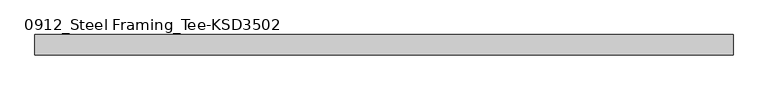
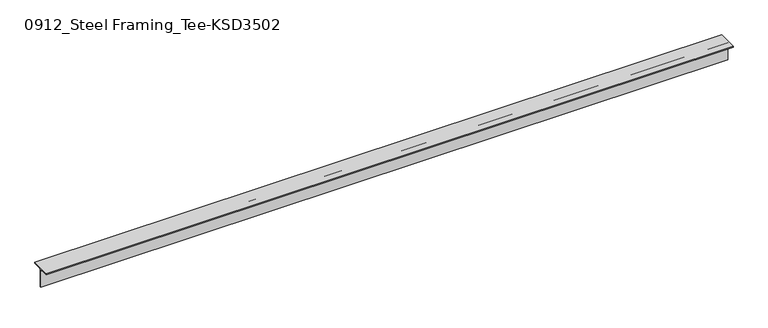
"""IFC4 building model written with IfcOpenShell, lengths in millimetres: member geometry, 0912_Steel Framing_Tee-KSD3502 : H_SB_ASB_CT-150x150x6.5x9."""

from ifc_helpers import new_model, si_unit, point, frame, frame_2d, origin, place, context, project, spatial, polyline, circle_curve, trimmed, segment, composite_curve, outline, extrude, source, transform, mapped, element, save


def member_0912_steel_framing_tee_ksd3502_70ece821(model_context):
    return source(origin(), model_context, "Body", "SweptSolid", [
        extrude(outline(composite_curve([segment(polyline([(-75.0, 75.0), (75.0, 75.0), (75.0, 66.0), (16.25, 66.0)]), True, "CONTINUOUS"), segment(trimmed(circle_curve(frame_2d((16.25, 53.0)), 13.0), [point((16.25, 66.0))], [point((3.25, 53.0))], True, "CARTESIAN"), True, "CONTINUOUS"), segment(polyline([(3.25, 53.0), (3.25, -75.0), (-3.25, -75.0), (-3.25, 53.0)]), True, "CONTINUOUS"), segment(trimmed(circle_curve(frame_2d((-16.25, 53.0)), 13.0), [point((-3.25, 53.0))], [point((-16.25, 66.0))], True, "CARTESIAN"), True, "CONTINUOUS"), segment(polyline([(-16.25, 66.0), (-75.0, 66.0), (-75.0, 75.0)]), True, "CONTINUOUS")], self_intersect=False)), frame((-2577.05, 0.0, 0.0), z_axis=(1.0, 0.0, 0.0), x_axis=(0.0, 1.0, 0.0)), (0.0, 0.0, 1.0), 5164.8),
    ])


if __name__ == "__main__":
    model = new_model("IFC4")
    model_context = context("Model", 3, world=origin())
    ifc_project = project(units=[si_unit("LENGTHUNIT", "METRE", prefix="MILLI")], contexts=[model_context])
    site = spatial("IfcSite", under=ifc_project)
    building = spatial("IfcBuilding", under=site)
    placement = place(None, origin())
    member_0912_steel_framing_tee_ksd3502_shape = member_0912_steel_framing_tee_ksd3502_70ece821(model_context)
    element("IfcMember", 1, ObjectType="0912_Steel Framing_Tee-KSD3502 : H_SB_ASB_CT-150x150x6.5x9", at=placement, inside=building, context=model_context, shape_type="MappedRepresentation", body=[
        mapped(member_0912_steel_framing_tee_ksd3502_shape, transform((0.0, 0.0, 0.0), x_axis=(1.0, 0.0, 0.0), y_axis=(0.0, 1.0, 0.0), z_axis=(0.0, 0.0, 1.0))),
    ])
    save(model, "model.ifc")

# Revit data of these elements
# Type "0912_Steel Framing_Tee-KSD3502 : H_SB_ASB_CT-150x150x6.5x9"
#   H_WM Code_1 = "S01AA003-00001 | Main Steel Structure Fabrication Work | Shelter/Building | Light Steel - Standard (30KG/M>Weight) | Material: (   )"
#   H_WM Code_2 = "S03AA029-00001 | Main Steel Structure Erection Work | Shelter/Building | Light Steel (30KG/M>Weight) | Material: (   )"
#   H_WM Code_3 = "S01AA010-00001 | Main Steel Structure Fabrication Work | Shelter/Building | Steel Painting/Coating | for Non-Fireproofed Steel Surface, Surface Preparation, Primer, Second & Final Coat | Material: (   )"
#   H_Q'ty Cal Type Tag = "SB-Q2"
#   Width = 15.0 cm
#   Web Thickness = 0.65 cm
#   Web Fillet = 1.3 cm
#   Section Area = 23.39 cm²
#   Perimeter = 0.60 m²/m
#   Nominal Weight = 18.40 kgf/m
#   Height = 15.0 cm
#   Flange Thickness = 0.9 cm
#   Centroid Vertical = 7.5 cm
#   Centroid Horizontal = 7.5 cm
#   Length [instance default] = 1.5000 m
#   Structural Material [instance default] = Steel, 45-345
#   Warping Constant = (empty or 0)
#   Torsional Moment of Inertia = 0
#   Section Name Key = ""
#   Plastic Modulus weak axis = 0
#   Plastic Modulus strong axis = 0
#   Moment of Inertia weak axis = 0
#   Moment of Inertia strong axis = 0
#   Elastic Modulus weak axis = 0
#   Elastic Modulus strong axis = 0
#   Bolt Spacing = 0
#   Assembly Code = ""
# Element 1 (IfcMember, "0912_Steel Framing_Tee-KSD3502 : H_SB_ASB_CT-150x150x6.5x9")
#   Structural Material = none
# Materials
#   "Steel, 45-345": class "Metal", colour RGB 189 187 185, transparency 0, Description = "Steel 345 MPa", Cost = 0
